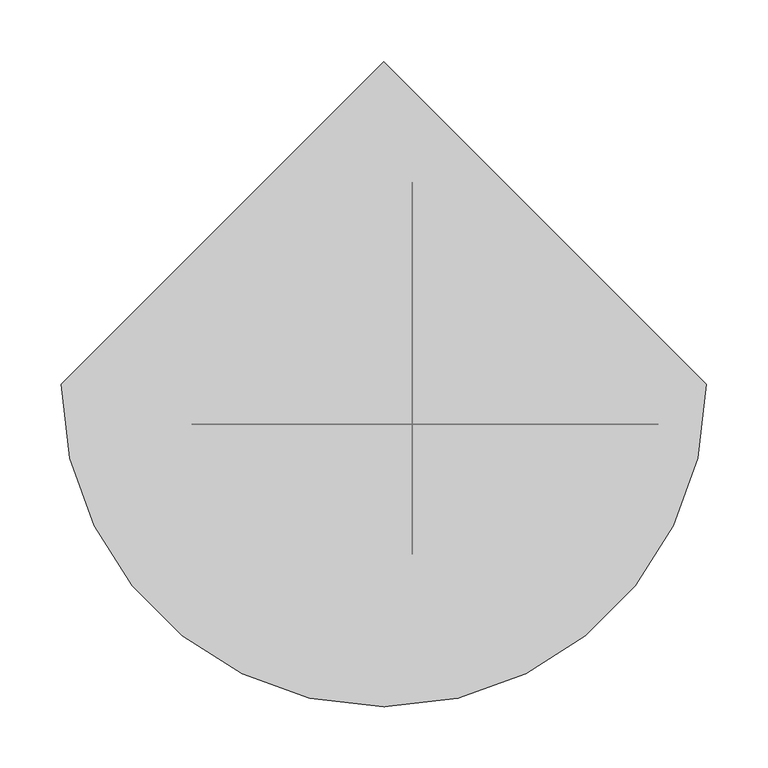
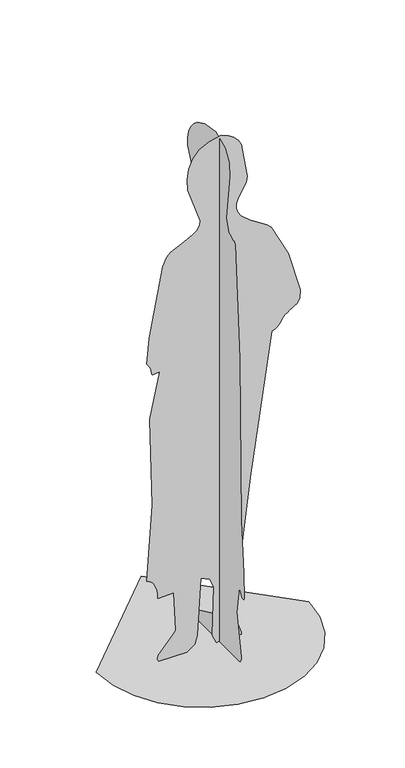
"""IFC4 building model written with IfcOpenShell, lengths in millimetres: proxy geometry, blaine 25105 : blaine 25105."""

from ifc_helpers import new_model, si_unit, origin, place, context, project, spatial, triangles, source, transform, mapped, element, save


def entourage_372d01d3(model_context):
    return source(origin(), model_context, "Body", "Tessellation", [
        triangles([(-126.0804764, -32.4912263, 3.89e-05), (-130.7749119, -32.4912263, 7.3726417), (-128.3293944, -32.4912263, 16.4650685), (-90.5836606, -32.4912263, 58.3741213), (-85.0147054, -32.4912263, 67.3217946), (-89.7683215, -32.4912263, 166.8800573), (-126.4421731, -32.4912263, 164.9745413), (-127.1325379, -32.4912263, 165.1322715), (-127.7891294, -32.4912263, 165.4119238), (-128.3347265, -32.4912263, 165.8414397), (-128.6913454, -32.4912263, 166.4492696), (-128.7812563, -32.4912263, 167.2635913), (-129.2382052, -32.4912263, 176.3931212), (-130.6771163, -32.4912263, 185.7116477), (-136.9105385, -32.4912263, 203.2361412), (-141.9097791, -32.4912263, 210.6021523), (-148.3006863, -32.4912263, 216.4774478), (-156.1851069, -32.4912263, 220.4421404), (-142.3260873, -32.4912263, 413.3323288), (-149.288998, -32.4912263, 640.3680347), (-124.0479606, -32.4912263, 756.0601736), (-142.0631945, -32.4912263, 754.1170509), (-142.669998, -32.4912263, 754.2644257), (-143.1698766, -32.4912263, 754.6301737), (-143.4929674, -32.4912263, 755.2879824), (-144.6301254, -32.4912263, 765.9610954), (-147.762456, -32.4912263, 774.6504633), (-156.1851069, -32.4912263, 786.0550724), (-150.0995136, -32.4912263, 852.2145515), (-116.4259149, -32.4912263, 1027.4952044), (-107.1759799, -32.4912263, 1048.3765606), (-97.3713095, -32.4912263, 1057.515465), (-70.2260369, -32.4912263, 1071.1553301), (-55.7449622, -32.4912263, 1077.4266043), (-42.5651344, -32.4912263, 1084.513163), (-32.1163195, -32.4912263, 1093.3041235), (-25.8287945, -32.4912263, 1104.6833708), (-24.5093393, -32.4912263, 1114.9043312), (-54.6583507, -32.4912263, 1204.9805191), (-56.7693455, -32.4912263, 1233.1110695), (-52.9004138, -32.4912263, 1259.2350563), (-42.7668118, -32.4912263, 1282.1458672), (-26.0840637, -32.4912263, 1300.6396511), (-2.5672329, -32.4912263, 1313.5022381), (28.0678089, -32.4912263, 1319.5321026), (45.292339, -32.4912263, 1312.5268616), (58.92124, -32.4912263, 1303.4640427), (69.3827517, -32.4912263, 1292.2296993), (77.1056406, -32.4912263, 1278.7066875), (92.0075835, -32.4912263, 1189.8700315), (89.3962058, -32.4912263, 1176.2556009), (68.5056886, -32.4912263, 1137.8354897), (65.2212097, -32.4912263, 1127.4189743), (64.7101626, -32.4912263, 1116.4689886), (67.9715279, -32.4912263, 1104.8840126), (76.0263869, -32.4912263, 1092.460861), (99.8094601, -32.4912263, 1072.9053686), (113.5701935, -32.4912263, 1064.4725985), (139.9110457, -32.4912263, 1047.0328926), (150.5236974, -32.4912263, 1036.7255276), (193.4347773, -32.4912263, 953.5835821), (223.2435137, -32.4912263, 848.6001646), (221.3593264, -32.4912263, 826.1592379), (218.1299632, -32.4912263, 820.1698505), (213.5429794, -32.4912263, 815.2473312), (208.0202424, -32.4912263, 811.0868294), (201.9834197, -32.4912263, 807.3809509), (195.8541245, -32.4912263, 803.8173603), (190.0537881, -32.4912263, 800.0936777), (185.0042599, -32.4912263, 795.8975676), (180.0954389, -32.4912263, 790.3045223), (176.3133659, -32.4912263, 784.9451111), (173.0301543, -32.4912263, 779.903195), (169.6181714, -32.4912263, 775.2651787), (165.4495123, -32.4912263, 771.1173214), (159.8965628, -32.4912263, 767.543557), (152.331672, -32.4912263, 764.6301447), (101.0459398, -32.4912263, 410.7212236), (56.9463832, -32.4912263, 62.9641618), (77.3959572, -32.4912263, 4.4354822), (77.5051801, -32.4912263, 3.89e-05), (15.5097739, -32.4912263, 3.89e-05), (5.0789159, -32.4912263, 22.3709592), (9.1479518, -32.4912263, 148.0710673), (-0.532903, -32.4912263, 170.4170144), (-23.3515293, -32.4912263, 181.8775067), (-31.3835291, -32.4909719, 35.6194942), (-38.3487266, -32.4909719, 14.7642821), (-58.0345209, -32.4912263, 3.89e-05), (23.1565058, -122.2049317, 1.937721), (23.1564808, -123.8221568, 4.5424928), (23.1564808, -124.8671148, 7.5824967), (23.1564808, -125.466297, 10.8258029), (23.1564808, -125.7451953, 14.0402029), (23.1564808, -125.8302828, 16.9941514), (23.1564808, -106.2112859, 121.1919848), (23.1564808, -117.2331331, 190.4474778), (23.1564808, -120.2242387, 189.0517417), (23.1564808, -122.1587045, 186.113985), (23.1564808, -125.164544, 178.2275115), (23.1564808, -127.3890811, 174.586927), (23.1564808, -130.8632968, 172.0205139), (23.1564808, -136.1640361, 171.182302), (23.1564808, -136.2549644, 171.7942014), (23.1564808, -138.4909289, 176.9730095), (23.1564808, -136.1487936, 241.0227701), (23.1564808, -125.1246663, 370.8609386), (23.1564808, -120.3959397, 790.6524662), (23.1565058, -99.2016392, 1077.1421013), (23.1565058, -98.8747424, 1078.3435541), (23.1565058, -98.410681, 1079.6287954), (23.1565058, -97.7629825, 1080.8403494), (23.1565058, -96.884902, 1081.8208128), (23.1565058, -95.7297127, 1082.4202675), (23.1565058, -94.2506606, 1082.476078), (23.1565058, -92.6895822, 1082.6437277), (23.1565058, -90.0715915, 1083.1568504), (23.1565058, -75.8777995, 1088.8439306), (23.1565058, -73.1117347, 1091.2238726), (23.1565058, -61.4955333, 1123.8756586), (23.1565058, -76.5387057, 1239.6769478), (23.1565058, -74.4716535, 1274.4749691), (23.1565058, -57.0081073, 1302.4912823), (23.1565058, -17.0341574, 1320.8022285), (23.1565058, 29.9278539, 1313.23801), (23.1565058, 63.3647233, 1296.6035603), (23.1565058, 78.2621016, 1283.8450367), (23.1565058, 90.6458933, 1268.6914558), (23.1565058, 99.5419982, 1251.5616875), (23.1565058, 103.97583, 1232.8850658), (23.1565058, 102.9730388, 1213.0780626), (23.1565058, 84.963137, 1175.585075), (23.1565058, 69.2925819, 1117.8812571), (23.1565058, 61.814559, 1105.6256824), (23.1565058, 51.9357198, 1095.5037712), (23.1565058, 39.1676265, 1088.1454268), (23.1565058, 17.742818, 1090.2866478), (23.1565058, 23.395699, 1051.9960344), (23.1565058, 36.6004435, 1013.352463), (23.1565058, 44.2748139, 993.9620768), (23.1565058, 51.7256627, 974.5615168), (23.1564808, 77.3972289, 881.127467), (23.1564808, 107.5930511, 843.0984655), (23.1564808, 108.9580477, 833.4337938), (23.1564808, 107.3141619, 825.0771818), (23.1564808, 91.3111143, 795.4378572), (23.1564808, 90.1183274, 786.659614), (23.1564808, 137.7215627, 640.3680347), (23.1564808, 139.1846093, 640.1851971), (23.1564808, 140.4744198, 639.5374895), (23.1564808, 141.5897405, 638.5011429), (23.1564808, 142.5292816, 637.1600183), (23.1564808, 143.2922983, 635.5878033), (23.1564808, 154.4462232, 569.4359181), (23.1564808, 155.5905029, 554.2492361), (23.1564808, 153.3443646, 539.3190791), (23.1564808, 146.2912886, 524.6734251), (23.1564808, 145.1858782, 524.3965525), (23.1564808, 135.9273045, 526.2812485), (23.1564808, 133.7972565, 526.2837919), (23.1564808, 132.2981474, 525.6106862), (23.1564808, 126.2028981, 497.4775924), (23.1564808, 164.0995039, 244.6511642), (23.1564808, 159.0123871, 220.1071136), (23.1564808, 21.6580053, 154.1244042), (23.1564808, -33.676644, 151.8828532), (23.1564808, -26.8201584, 87.1071558), (23.1564808, -18.4245556, 69.3936749), (23.1564808, -13.0358345, 62.9049812), (23.1564808, -3.5679945, 55.9499415), (23.1564558, 50.5938368, 30.6807104), (23.1564558, 63.6819687, 19.2270195), (23.1564558, 74.7792473, 3.4089903), (23.1564558, 75.1290034, 3.0369561), (23.1564558, 75.4454903, 2.4998491), (23.1564808, 75.659358, 1.8737407), (23.1564808, 75.7010161, 1.2346833), (23.1564808, 75.5011146, 0.6585926), (23.1564808, 74.9903218, 0.2217434), (23.1565058, 74.0990336, 4.52e-05), (23.1565058, -119.8894662, 3.37e-05), (-262.2401886, -2.2e-06, 4.08e-05), (-255.3059825, -60.0878612, 3.72e-05), (-235.5620205, -115.2689452, 3.39e-05), (-204.5869127, -163.9623393, 3.1e-05), (-163.9623393, -204.5869127, 2.86e-05), (-115.2689452, -235.5620205, 2.68e-05), (-60.0878612, -255.3059825, 2.56e-05), (1.15e-05, -262.2401886, 2.52e-05), (60.0878612, -255.3059825, 2.56e-05), (115.2689452, -235.5620205, 2.68e-05), (163.9623393, -204.5869127, 2.86e-05), (204.587167, -163.9623393, 3.1e-05), (235.5620205, -115.2689452, 3.39e-05), (255.3059825, -60.0878612, 3.72e-05), (262.2401886, 2.08e-05, 4.08e-05), (-3.45e-05, 262.2401886, 5.64e-05)], [[80, 81, 82], [80, 82, 83], [79, 80, 83], [79, 83, 84], [78, 79, 84], [78, 84, 85], [17, 18, 19], [78, 85, 86], [89, 1, 2], [89, 2, 3], [88, 89, 3], [88, 3, 4], [87, 88, 4], [87, 4, 5], [87, 5, 6], [86, 87, 6], [16, 17, 19], [78, 86, 6], [78, 6, 7], [78, 7, 8], [78, 8, 9], [78, 9, 10], [78, 10, 11], [78, 11, 12], [78, 12, 13], [78, 13, 14], [78, 14, 15], [78, 15, 16], [78, 16, 19], [78, 19, 20], [78, 20, 21], [77, 78, 21], [44, 45, 46], [44, 46, 47], [43, 44, 47], [43, 47, 48], [43, 48, 49], [42, 43, 49], [41, 42, 49], [40, 41, 49], [39, 40, 49], [39, 49, 50], [39, 50, 51], [39, 51, 52], [39, 52, 53], [38, 39, 53], [38, 53, 54], [37, 38, 54], [37, 54, 55], [36, 37, 55], [36, 55, 56], [35, 36, 56], [35, 56, 57], [34, 35, 57], [34, 57, 58], [33, 34, 58], [33, 58, 59], [33, 59, 60], [33, 60, 61], [32, 33, 61], [31, 32, 61], [30, 31, 61], [29, 30, 61], [29, 61, 62], [29, 62, 63], [29, 63, 64], [29, 64, 65], [29, 65, 66], [29, 66, 67], [29, 67, 68], [29, 68, 69], [29, 69, 70], [29, 70, 71], [29, 71, 72], [29, 72, 73], [29, 73, 74], [29, 74, 75], [29, 75, 76], [29, 76, 77], [29, 77, 21], [28, 29, 21], [27, 28, 21], [26, 27, 21], [25, 26, 21], [25, 21, 22], [24, 25, 22], [24, 22, 23], [102, 103, 104], [163, 164, 165], [101, 102, 104], [100, 101, 104], [100, 104, 105], [100, 105, 106], [99, 100, 106], [98, 99, 106], [97, 98, 106], [156, 157, 158], [156, 158, 159], [155, 156, 159], [155, 159, 160], [154, 155, 160], [154, 160, 161], [180, 181, 90], [180, 90, 91], [180, 91, 92], [180, 92, 93], [180, 93, 94], [180, 94, 95], [180, 95, 96], [179, 180, 96], [178, 179, 96], [177, 178, 96], [176, 177, 96], [175, 176, 96], [174, 175, 96], [173, 174, 96], [162, 163, 165], [162, 165, 166], [135, 136, 137], [134, 135, 137], [133, 134, 137], [123, 124, 125], [122, 123, 125], [121, 122, 125], [121, 125, 126], [121, 126, 127], [121, 127, 128], [121, 128, 129], [121, 129, 130], [121, 130, 131], [121, 131, 132], [121, 132, 133], [121, 133, 137], [120, 121, 137], [119, 120, 137], [119, 137, 138], [118, 119, 138], [118, 138, 139], [117, 118, 139], [116, 117, 139], [116, 139, 140], [115, 116, 140], [115, 140, 141], [114, 115, 141], [113, 114, 141], [112, 113, 141], [111, 112, 141], [110, 111, 141], [109, 110, 141], [109, 141, 142], [108, 109, 142], [108, 142, 143], [108, 143, 144], [108, 144, 145], [108, 145, 146], [108, 146, 147], [108, 147, 148], [107, 108, 148], [107, 148, 149], [107, 149, 150], [107, 150, 151], [107, 151, 152], [107, 152, 153], [107, 153, 154], [107, 154, 161], [107, 161, 162], [107, 162, 166], [106, 107, 166], [97, 106, 166], [96, 97, 166], [96, 166, 167], [96, 167, 168], [96, 168, 169], [171, 172, 173], [170, 171, 173], [170, 173, 96], [170, 96, 169], [196, 197, 182], [195, 196, 182], [195, 182, 183], [194, 195, 183], [194, 183, 184], [194, 184, 185], [193, 194, 185], [192, 193, 185], [192, 185, 186], [192, 186, 187], [192, 187, 188], [192, 188, 189], [192, 189, 190], [192, 190, 191]], closed=False),
    ])


if __name__ == "__main__":
    model = new_model("IFC4")
    model_context = context("Model", 3, world=origin())
    ifc_project = project(units=[si_unit("LENGTHUNIT", "METRE", prefix="MILLI")], contexts=[model_context])
    site = spatial("IfcSite", under=ifc_project)
    building = spatial("IfcBuilding", under=site)
    placement = place(None, origin())
    entourage_shape = entourage_372d01d3(model_context)
    element("IfcBuildingElementProxy", 1, Name="blaine 25105 : blaine 25105", ObjectType="blaine 25105 : blaine 25105", at=placement, inside=building, context=model_context, shape_type="MappedRepresentation", body=[
        mapped(entourage_shape, transform((0.0, 0.0, 0.0), x_axis=(1.0, 0.0, 0.0), y_axis=(0.0, 1.0, 0.0), z_axis=(0.0, 0.0, 1.0))),
    ])
    save(model, "model.ifc")

# Revit data of these elements
# Type "blaine 25105 : blaine 25105"
#   built-in parameter 1005195 = "RPC-8-G3GR-0A00-PN13-W"
#   Height = 0
